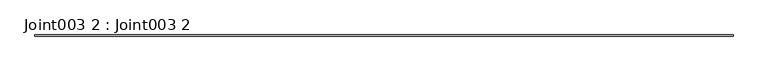
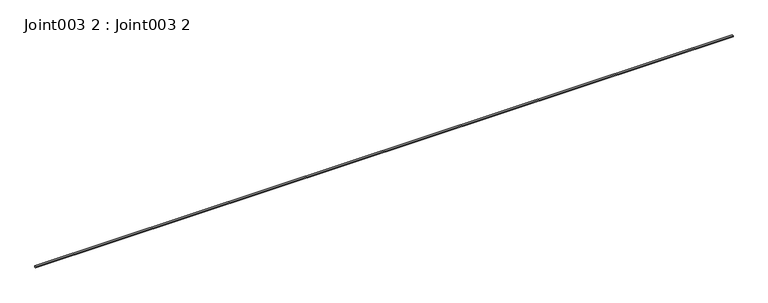
"""IFC4 building model written with IfcOpenShell, lengths in millimetres: proxy geometry, Joint003 2 : Joint003 2."""

from ifc_helpers import new_model, si_unit, point, frame, frame_2d, origin, place, context, project, spatial, polyline, circle_curve, trimmed, segment, composite_curve, outline, extrude, source, transform, mapped, element, save


def joint003_2_joint003_2_9bc8abc8(model_context):
    return source(origin(), model_context, "Body", "SweptSolid", [
        extrude(outline(composite_curve([segment(polyline([(9721.6885026, 39516.5389688), (9721.6885026, 39512.621)]), True, "CONTINUOUS"), segment(trimmed(circle_curve(frame_2d((9720.0901706, 39507.449125)), 5.4132205), [point((9721.6885026, 39512.621))], [point((9718.4918386, 39512.621))], True, "CARTESIAN"), True, "CONTINUOUS"), segment(polyline([(9718.4918386, 39512.621), (9718.4918386, 39516.5389688)]), True, "CONTINUOUS"), segment(trimmed(circle_curve(frame_2d((9720.0901706, 39511.3670938)), 5.4132205), [point((9718.4918386, 39516.5389688))], [point((9721.6885026, 39516.5389688))], False, "CARTESIAN"), True, "CONTINUOUS")], self_intersect=False)), frame((3694.2883192, 0.0, 0.0), z_axis=(1.0, 0.0, 0.0), x_axis=(0.0, 1.0, 0.0)), (0.0, 0.0, 1.0), 2000.0),
    ])


if __name__ == "__main__":
    model = new_model("IFC4")
    model_context = context("Model", 3, world=origin())
    ifc_project = project(units=[si_unit("LENGTHUNIT", "METRE", prefix="MILLI")], contexts=[model_context])
    site = spatial("IfcSite", under=ifc_project)
    building = spatial("IfcBuilding", under=site)
    placement = place(None, origin())
    joint003_2_joint003_2_shape = joint003_2_joint003_2_9bc8abc8(model_context)
    element("IfcBuildingElementProxy", 1, Name="Joint003 2 : Joint003 2", ObjectType="Joint003 2 : Joint003 2", at=placement, inside=building, context=model_context, shape_type="MappedRepresentation", body=[
        mapped(joint003_2_joint003_2_shape, transform((0.0, 0.0, 0.0), x_axis=(1.0, 0.0, 0.0), y_axis=(0.0, 1.0, 0.0), z_axis=(0.0, 0.0, 1.0))),
    ])
    save(model, "model.ifc")

# Revit data of these elements
# Type "Joint003 2 : Joint003 2"
#   NameOverride = "Joint003"
# Element 1 (IfcBuildingElementProxy, "Joint003 2 : Joint003 2")
#   Materials on its faces: "SEALANT JOINT"
# Materials
#   "SEALANT JOINT": class "Unassigned", colour RGB 142 225 148, transparency 0
